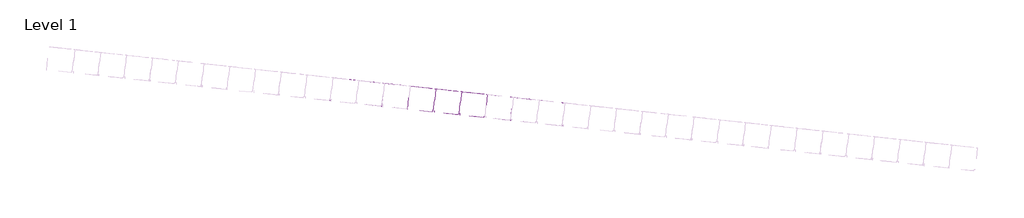
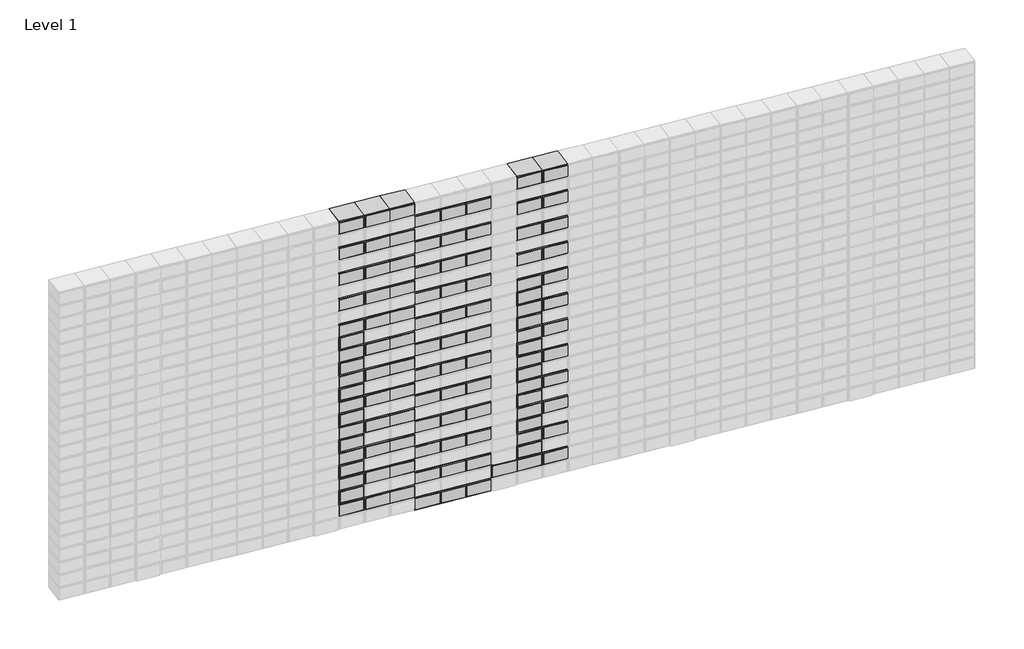
# One storey, part 14 of 18: 111 proxies.
# Revit data of these elements (continued)
# Elements 62, 63, 64, 65, 66, 67, 68, 69, 70, 71, 72, 73 (IfcBuildingElementProxy, "00_GMA_steen_versie_6 : Rood") (continued)
#   Materials on its faces: "20_voeg", "21_steen_rood"
# Elements 74, 75, 76, 77, 78, 79, 80, 81, 82, 83, 84, 85, 86, 87, 88, 89, 90, 91, 92, 93, 94, 95, 96, 97, 98, 99, 100, 101, 102, 103, 104, 105, 106, 107, 108, 109, 110, 111 (IfcBuildingElementProxy, "00_GMA_steen_versie_6 : Rood")
#   StootvoegLinksHalfOnder = 5 mm
#   StootvoegLinksHalfBoven = 5 mm
#   StootVoegRechtsHalfOnder = 5 mm
#   StootVoegRechtsHalfBoven = 5 mm
#   StootVoegBreedteRechts = 10 mm
#   StootVoegBreedteLinks = 10 mm
#   LintVoegOnderHalf = 5 mm
#   LintVoegOnder = 10 mm
#   LintVoegBovenHalf = 5 mm
#   LintVoegBoven = 10 mm
#   Phase Created = New Construction
#   Materials on its faces: "20_voeg", "21_steen_rood"
# Materials
#   "21_steen_geel": class "Unassigned", colour RGB 202 202 0, transparency 0, Cost = 0
#   "20_voeg": class "Concrete", colour RGB 86 86 86, transparency 0, Manufacturer = "RevitGG", URL = "www.revitgg.nl", Description = "zandcement, generiek materiaal", Cost = 0
#   "21_steen_rood": class "Unassigned", colour RGB 213 111 43, transparency 0, Cost = 0
